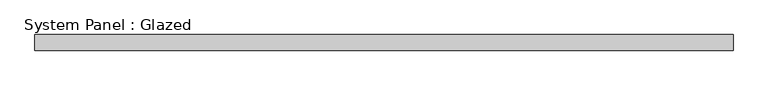
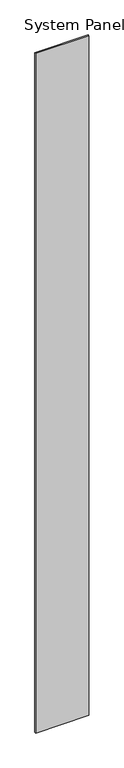
"""IFC4 building model written with IfcOpenShell, lengths in millimetres: plate geometry, System Panel : Glazed."""

import ifcopenshell
import ifcopenshell.guid

model = None  # the IFC model being written
_history = None  # IfcOwnerHistory: only IFC2X3 demands one
_inside = {}  # id of a spatial element -> (the spatial element, [elements in it])
_under = {}  # id of a project, library or spatial element -> (it, [spatial elements below it])
_declared = {}  # id of a project -> (the project, [libraries it declares])
_typed = {}  # id of a type object -> (the type object, [elements of that type])
_made_of = {}  # id of a material, layer set ... -> (it, [elements and type objects made of it])


def new_model(schema):
    """Start an empty IFC model of exactly this schema.

    Asked for "IFC4X3", IfcOpenShell would pick the latest addendum, in which some entities
    have other attributes; the version numbers below select the first issue.
    IFC2X3 requires an IfcOwnerHistory on every rooted entity: one is made here for all.
    """
    global model, _history
    if schema == "IFC4X3":
        model = ifcopenshell.file(schema_version=(4, 3, 0, 0))
    else:
        model = ifcopenshell.file(schema=schema)
    _inside.clear()
    _under.clear()
    _declared.clear()
    _typed.clear()
    _made_of.clear()
    _history = None
    if model.schema == "IFC2X3":
        org = make("IfcOrganization", Name="unknown")
        user = make(
            "IfcPersonAndOrganization",
            ThePerson=make("IfcPerson", FamilyName="unknown"),
            TheOrganization=org,
        )
        app = make(
            "IfcApplication",
            ApplicationDeveloper=org,
            Version="unknown",
            ApplicationFullName="unknown",
            ApplicationIdentifier="unknown",
        )
        _history = make(
            "IfcOwnerHistory",
            OwningUser=user,
            OwningApplication=app,
            ChangeAction="ADDED",
            CreationDate=0,
        )
    return model


def make(cls, **values):
    """One entity of the class cls with the attributes given. An attribute that is None is left unset."""
    return model.create_entity(
        cls, **{name: value for name, value in values.items() if value is not None}
    )


def rooted(cls, **values):
    """An entity with a GlobalId (a new one), such as an element, a storey or a relation."""
    return make(cls, GlobalId=ifcopenshell.guid.new(), OwnerHistory=_history, **values)


def si_unit(unit_type, name, prefix=None):
    """IfcSIUnit, for example si_unit("LENGTHUNIT", "METRE", prefix="MILLI")."""
    return make("IfcSIUnit", UnitType=unit_type, Prefix=prefix, Name=name)


def assignment(units):
    """IfcUnitAssignment: the units of a project."""
    return None if units is None else make("IfcUnitAssignment", Units=units)


def point(xyz):
    """IfcCartesianPoint."""
    return None if xyz is None else make("IfcCartesianPoint", Coordinates=xyz)


def direction(xyz):
    """IfcDirection."""
    return None if xyz is None else make("IfcDirection", DirectionRatios=xyz)


def frame(location, z_axis=None, x_axis=None):
    """IfcAxis2Placement3D, a coordinate frame: its origin and axes. An axis left out is left unset."""
    return make(
        "IfcAxis2Placement3D",
        Location=point(location),
        Axis=direction(z_axis),
        RefDirection=direction(x_axis),
    )


def origin():
    """The frame at (0, 0, 0) with its axes left unset."""
    return frame((0.0, 0.0, 0.0))


def origin_with_axes():
    """The frame at (0, 0, 0) with the z axis (0, 0, 1) and the x axis (1, 0, 0) written out."""
    return frame((0.0, 0.0, 0.0), z_axis=(0.0, 0.0, 1.0), x_axis=(1.0, 0.0, 0.0))


def place(relative_to, where):
    """IfcLocalPlacement: puts the frame where relative to a parent placement (None: the world)."""
    return make(
        "IfcLocalPlacement", PlacementRelTo=relative_to, RelativePlacement=where
    )


def context(
    kind, dimensions, precision=None, world=None, true_north=None, identifier=None
):
    """IfcGeometricRepresentationContext, for example the 3D "Model" context."""
    return make(
        "IfcGeometricRepresentationContext",
        ContextIdentifier=identifier,
        ContextType=kind,
        CoordinateSpaceDimension=dimensions,
        Precision=precision,
        WorldCoordinateSystem=world,
        TrueNorth=true_north,
    )


def project(units=None, contexts=None):
    """IfcProject with its units and contexts."""
    return rooted(
        "IfcProject",
        Name="project",
        RepresentationContexts=contexts,
        UnitsInContext=assignment(units),
    )


def spatial(cls, under=None, at=None, **own):
    """A site, building, storey or space (cls), placed at a placement, below another one or the project."""
    s = rooted(cls, ObjectPlacement=at, **own)
    if under is not None:
        _under.setdefault(under.id(), (under, []))[1].append(s)
    return s


def polyline(points):
    """IfcPolyline through the points."""
    return make("IfcPolyline", Points=[point(p) for p in points])


def outline(outer, holes=None, kind="AREA"):
    """IfcArbitraryClosedProfileDef: a profile drawn as a closed curve; with holes, ...WithVoids."""
    if holes is None:
        return make("IfcArbitraryClosedProfileDef", ProfileType=kind, OuterCurve=outer)
    return make(
        "IfcArbitraryProfileDefWithVoids",
        ProfileType=kind,
        OuterCurve=outer,
        InnerCurves=holes,
    )


def extrude(swept, where, along, depth):
    """IfcExtrudedAreaSolid: the profile swept, set in the frame where, extruded along a direction by depth."""
    return make(
        "IfcExtrudedAreaSolid",
        SweptArea=swept,
        Position=where,
        ExtrudedDirection=direction(along),
        Depth=depth,
    )


def shape(context_of_items, identifier, shape_type, items):
    """IfcShapeRepresentation: the items that make up one representation, for example the "Body"."""
    return make(
        "IfcShapeRepresentation",
        ContextOfItems=context_of_items,
        RepresentationIdentifier=identifier,
        RepresentationType=shape_type,
        Items=items,
    )


def source(mapping_origin, context_of_items, identifier, shape_type, items):
    """IfcRepresentationMap: a shape defined once, which mapped items show again and again."""
    return make(
        "IfcRepresentationMap",
        MappingOrigin=mapping_origin,
        MappedRepresentation=shape(context_of_items, identifier, shape_type, items),
    )


def transform(
    local_origin,
    x_axis=None,
    y_axis=None,
    z_axis=None,
    scale=None,
    scale2=None,
    scale3=None,
    uniform=True,
):
    """IfcCartesianTransformationOperator3D, or its non-uniform kind. x_axis, y_axis, z_axis: its Axis1, 2, 3."""
    if uniform:
        return make(
            "IfcCartesianTransformationOperator3D",
            Axis1=direction(x_axis),
            Axis2=direction(y_axis),
            LocalOrigin=point(local_origin),
            Scale=scale,
            Axis3=direction(z_axis),
        )
    return make(
        "IfcCartesianTransformationOperator3DnonUniform",
        Axis1=direction(x_axis),
        Axis2=direction(y_axis),
        LocalOrigin=point(local_origin),
        Scale=scale,
        Axis3=direction(z_axis),
        Scale2=scale2,
        Scale3=scale3,
    )


def mapped(mapping_source, mapping_target):
    """IfcMappedItem: shows the shape of a source again, moved by a transform."""
    return make(
        "IfcMappedItem", MappingSource=mapping_source, MappingTarget=mapping_target
    )


def made_of(thing, what):
    """Note that an element or type object is made of a material, layer set ...; save() writes the relation."""
    if what is not None:
        _made_of.setdefault(what.id(), (what, []))[1].append(thing)
    return thing


def element(
    cls,
    number,
    at=None,
    inside=None,
    cuts=None,
    type_object=None,
    material=None,
    context=None,
    identifier="Body",
    shape_type=None,
    held_by="IfcProductDefinitionShape",
    body=None,
    shapes=None,
    **own,
):
    """One element of the class cls, such as IfcWall. Its Tag is "e" and its number.

    at: its placement. inside: the storey or other place that contains it. cuts: it is an
    opening in that element (IfcRelVoidsElement). A single representation is given by context,
    identifier, shape_type and body (its items); several are given by shapes. held_by: the class
    of the entity that holds the representations. save() writes the other relations.
    """
    e = rooted(cls, Tag="e%d" % number, ObjectPlacement=at, **own)
    if body is not None:
        shapes = [shape(context, identifier, shape_type, body)]
    if shapes is not None:
        e.Representation = make(held_by, Representations=shapes)
    if inside is not None:
        _inside.setdefault(inside.id(), (inside, []))[1].append(e)
    if cuts is not None:
        rooted(
            "IfcRelVoidsElement", RelatingBuildingElement=cuts, RelatedOpeningElement=e
        )
    if type_object is not None:
        _typed.setdefault(type_object.id(), (type_object, []))[1].append(e)
    return made_of(e, material)


def aggregate(whole, parts):
    """IfcRelAggregates: a whole, such as a stair, and the parts it consists of."""
    return rooted("IfcRelAggregates", RelatingObject=whole, RelatedObjects=parts)


def save(model, path):
    """Write the relations noted so far, then the file.

    IfcRelAggregates (storeys below a building ...), IfcRelContainedInSpatialStructure (elements
    in a storey), IfcRelDefinesByType, IfcRelAssociatesMaterial and IfcRelDeclares: one each for
    every whole, place, type object, material and project.
    """
    for whole, parts in _under.values():
        aggregate(whole, parts)
    for where, things in _inside.values():
        rooted(
            "IfcRelContainedInSpatialStructure",
            RelatedElements=things,
            RelatingStructure=where,
        )
    for kind, things in _typed.values():
        rooted("IfcRelDefinesByType", RelatedObjects=things, RelatingType=kind)
    for what, things in _made_of.values():
        rooted("IfcRelAssociatesMaterial", RelatedObjects=things, RelatingMaterial=what)
    for by, libraries in _declared.values():
        rooted("IfcRelDeclares", RelatingContext=by, RelatedDefinitions=libraries)
    model.write(path)


def system_panel_glazed_21f2c726(model_context):
    return source(origin(), model_context, "Body", "SweptSolid", [
        extrude(outline(polyline([(553.4450969, 19.05), (-553.4450969, 19.05), (-553.4450969, 44.45), (553.4450969, 44.45), (553.4450969, 19.05)])), origin_with_axes(), (0.0, 0.0, 1.0), 14960.6),
    ])


if __name__ == "__main__":
    model = new_model("IFC4")
    model_context = context("Model", 3, world=origin())
    ifc_project = project(units=[si_unit("LENGTHUNIT", "METRE", prefix="MILLI")], contexts=[model_context])
    site = spatial("IfcSite", under=ifc_project)
    building = spatial("IfcBuilding", under=site)
    placement = place(None, origin())
    system_panel_glazed_shape = system_panel_glazed_21f2c726(model_context)
    element("IfcPlate", 1, ObjectType="System Panel : Glazed", at=placement, inside=building, context=model_context, shape_type="MappedRepresentation", body=[
        mapped(system_panel_glazed_shape, transform((0.0, 0.0, 0.0), x_axis=(1.0, 0.0, 0.0), y_axis=(0.0, 1.0, 0.0), z_axis=(0.0, 0.0, 1.0))),
    ])
    save(model, "model.ifc")

# Revit data of these elements
# Type "System Panel : Glazed"
#   Construction Type Id = "GSP4R"
#   Analytic Construction = "1/8 in Pilkington single glazing"
#   Visual Light Transmittance = 0.9
#   Solar Heat Gain Coefficient = 0.86
#   Heat Transfer Coefficient (U) = 1.18115 BTU/(h·ft²·°F)
#   Define Thermal Properties by = 1
# Element 1 (IfcPlate, "System Panel : Glazed")
#   Materials on its faces: "Glass"
# Materials
#   "Glass": class "Glass", colour RGB 0 128 192, transparency 0.75, Description = "Soda Lime Glass", Cost = 0
